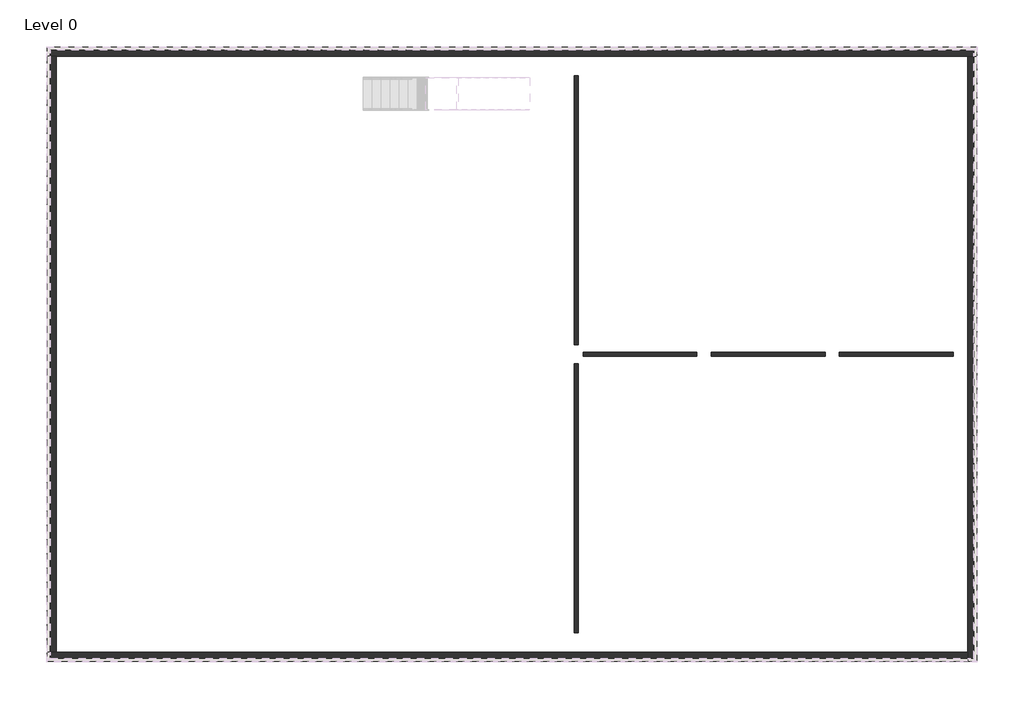
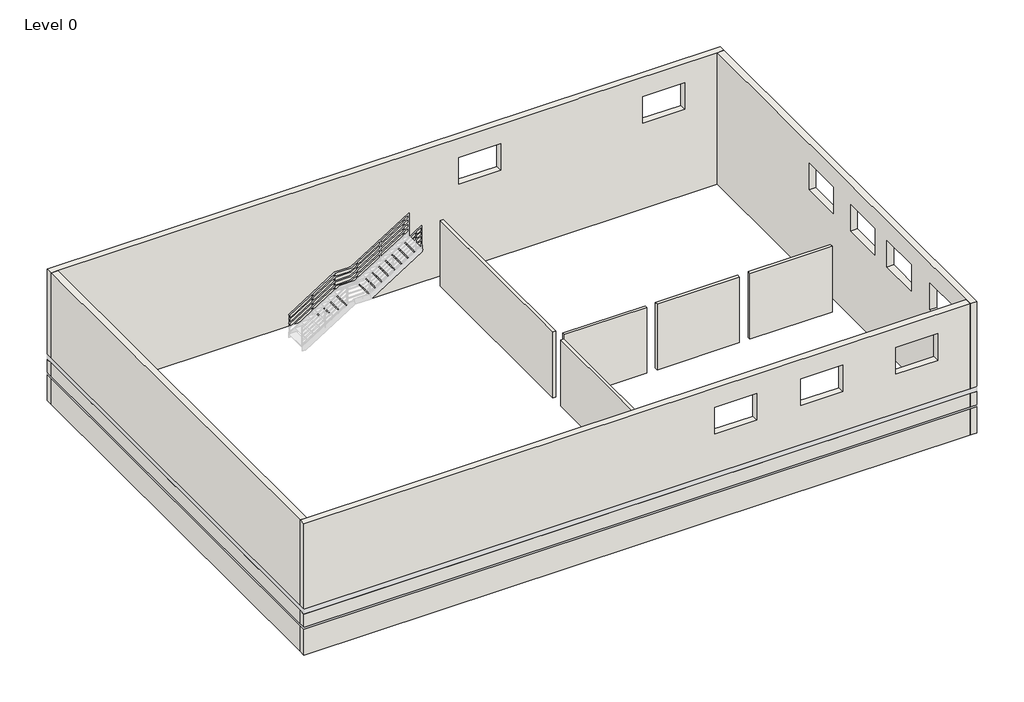
# One storey, part 1 of 3: 9 walls.
"""IFC4 building model written with IfcOpenShell, lengths in millimetres."""

from ifc_helpers import new_model, si_unit, frame, origin, origin_with_axes, place, context, project, spatial, polyline, outline, extrude, faceted_brep, element, save

model = new_model("IFC4")

# Units and contexts
model_context = context("Model", 3, world=origin())
ifc_project = project(units=[si_unit("LENGTHUNIT", "METRE", prefix="MILLI")], contexts=[model_context])

# Site, building, storey
site = spatial("IfcSite", under=ifc_project)
building = spatial("IfcBuilding", under=site)
storey = spatial("IfcBuildingStorey", under=building, Name="Level 0", Elevation=0.0)

# Walls
placement = place(None, origin())
element("IfcWall", 1, ObjectType="Wall-Ext_102Bwk-75Ins-100Blk-12P_Banding", at=placement, inside=storey, context=model_context, shape_type="Brep", body=[
    faceted_brep([(-15731.2051668, 9883.1317199, 0.0), (-15441.2051668, 9883.1317199, 0.0), (13008.7948332, 9883.1317199, 0.0), (13298.7948332, 9883.1317199, 0.0), (13298.7948332, 9883.1317199, 1200.0), (13216.2948332, 9883.1317199, 1200.0), (13216.2948332, 9883.1317199, 1275.0), (13298.7948332, 9883.1317199, 1275.0), (13298.7948332, 9883.1317199, 1885.0), (13196.7948332, 9883.1317199, 1885.0), (13196.7948332, 9883.1317199, 2110.0), (13298.7948332, 9883.1317199, 2110.0), (13298.7948332, 9883.1317199, 6000.0), (13008.7948332, 9883.1317199, 6000.0), (7058.7948332, 9883.1317199, 6000.0), (6958.7948332, 9883.1317199, 6000.0), (-15441.2051668, 9883.1317199, 6000.0), (-15731.2051668, 9883.1317199, 6000.0), (-15731.2051668, 9883.1317199, 2110.0), (-15629.2051668, 9883.1317199, 2110.0), (-15629.2051668, 9883.1317199, 1885.0), (-15731.2051668, 9883.1317199, 1885.0), (-15731.2051668, 9883.1317199, 1275.0), (-15648.7051668, 9883.1317199, 1275.0), (-15648.7051668, 9883.1317199, 1200.0), (-15731.2051668, 9883.1317199, 1200.0), (1848.7948332, 9883.1317199, 3900.0), (1848.7948332, 9883.1317199, 5110.0), (3658.7948332, 9883.1317199, 5110.0), (3658.7948332, 9883.1317199, 3900.0), (9798.7948332, 9883.1317199, 3900.0), (9798.7948332, 9883.1317199, 5110.0), (11608.7948332, 9883.1317199, 5110.0), (11608.7948332, 9883.1317199, 3900.0), (13298.7948332, 10173.1317199, 0.0), (-15731.2051668, 10173.1317199, 0.0), (-15731.2051668, 10173.1317199, 1200.0), (13298.7948332, 10173.1317199, 1200.0), (-15731.2051668, 10173.1317199, 6000.0), (13298.7948332, 10173.1317199, 6000.0), (13298.7948332, 10173.1317199, 2110.0), (-15731.2051668, 10173.1317199, 2110.0), (1848.7948332, 10173.1317199, 5110.0), (1848.7948332, 10173.1317199, 3900.0), (3658.7948332, 10173.1317199, 3900.0), (3658.7948332, 10173.1317199, 5110.0), (9798.7948332, 10173.1317199, 5110.0), (9798.7948332, 10173.1317199, 3900.0), (11608.7948332, 10173.1317199, 3900.0), (11608.7948332, 10173.1317199, 5110.0), (13298.7948332, 10173.1317199, 1275.0), (-15731.2051668, 10173.1317199, 1275.0), (-15731.2051668, 10173.1317199, 1885.0), (13298.7948332, 10173.1317199, 1885.0), (-15648.7051668, 10090.6317199, 1200.0), (-15648.7051668, 10090.6317199, 1275.0), (13216.2948332, 10090.6317199, 1275.0), (13216.2948332, 10090.6317199, 1200.0), (-15629.2051668, 10071.1317199, 1885.0), (-15629.2051668, 10071.1317199, 2110.0), (13196.7948332, 10071.1317199, 2110.0), (13196.7948332, 10071.1317199, 1885.0)], [[[0, 1, 2, 3, 4, 5, 6, 7, 8, 9, 10, 11, 12, 13, 14, 15, 16, 17, 18, 19, 20, 21, 22, 23, 24, 25], [26, 27, 28, 29], [30, 31, 32, 33]], [[34, 35, 36, 37]], [[38, 39, 40, 41], [42, 43, 44, 45], [46, 47, 48, 49]], [[50, 51, 52, 53]], [[3, 2, 1, 0, 35, 34]], [[17, 16, 15, 14, 13, 12, 39, 38]], [[54, 55, 56, 57]], [[58, 59, 60, 61]], [[3, 34, 37, 4]], [[39, 12, 11, 40]], [[7, 50, 53, 8]], [[57, 56, 6, 5]], [[61, 60, 10, 9]], [[17, 38, 41, 18]], [[35, 0, 25, 36]], [[51, 22, 21, 52]], [[55, 54, 24, 23]], [[56, 55, 23, 22, 51, 50, 7, 6]], [[54, 57, 5, 4, 37, 36, 25, 24]], [[59, 58, 20, 19]], [[60, 59, 19, 18, 41, 40, 11, 10]], [[58, 61, 9, 8, 53, 52, 21, 20]], [[43, 42, 27, 26]], [[44, 43, 26, 29]], [[45, 44, 29, 28]], [[42, 45, 28, 27]], [[47, 46, 31, 30]], [[48, 47, 30, 33]], [[49, 48, 33, 32]], [[46, 49, 32, 31]]]),
])
element("IfcWall", 2, ObjectType="Wall-Ext_102Bwk-75Ins-100Blk-12P_Banding", at=placement, inside=storey, context=model_context, shape_type="Brep", body=[
    faceted_brep([(13008.7948332, 9883.1317199, 0.0), (13008.7948332, -8716.8682801, 0.0), (13008.7948332, -9006.8682801, 0.0), (13008.7948332, -9006.8682801, 1200.0), (13008.7948332, -8924.3682801, 1200.0), (13008.7948332, -8924.3682801, 1275.0), (13008.7948332, -9006.8682801, 1275.0), (13008.7948332, -9006.8682801, 1885.0), (13008.7948332, -8904.8682801, 1885.0), (13008.7948332, -8904.8682801, 2110.0), (13008.7948332, -9006.8682801, 2110.0), (13008.7948332, -9006.8682801, 6000.0), (13008.7948332, -8716.8682801, 6000.0), (13008.7948332, 5333.1317199, 6000.0), (13008.7948332, 5433.1317199, 6000.0), (13008.7948332, 9883.1317199, 6000.0), (13008.7948332, -6006.8682801, 3900.0), (13008.7948332, -6006.8682801, 5110.0), (13008.7948332, -7816.8682801, 5110.0), (13008.7948332, -7816.8682801, 3900.0), (13008.7948332, -2796.8682801, 3900.0), (13008.7948332, -2796.8682801, 5110.0), (13008.7948332, -4606.8682801, 5110.0), (13008.7948332, -4606.8682801, 3900.0), (13008.7948332, -86.8682801, 3900.0), (13008.7948332, -86.8682801, 5110.0), (13008.7948332, -1896.8682801, 5110.0), (13008.7948332, -1896.8682801, 3900.0), (13008.7948332, 3023.1317199, 3900.0), (13008.7948332, 3023.1317199, 5110.0), (13008.7948332, 1213.1317199, 5110.0), (13008.7948332, 1213.1317199, 3900.0), (13298.7948332, -9006.8682801, 0.0), (13298.7948332, 9883.1317199, 0.0), (13298.7948332, 9883.1317199, 1200.0), (13298.7948332, -9006.8682801, 1200.0), (13298.7948332, 9883.1317199, 6000.0), (13298.7948332, -9006.8682801, 6000.0), (13298.7948332, -9006.8682801, 2110.0), (13298.7948332, 9883.1317199, 2110.0), (13298.7948332, -6006.8682801, 5110.0), (13298.7948332, -6006.8682801, 3900.0), (13298.7948332, -7816.8682801, 3900.0), (13298.7948332, -7816.8682801, 5110.0), (13298.7948332, -2796.8682801, 5110.0), (13298.7948332, -2796.8682801, 3900.0), (13298.7948332, -4606.8682801, 3900.0), (13298.7948332, -4606.8682801, 5110.0), (13298.7948332, -86.8682801, 5110.0), (13298.7948332, -86.8682801, 3900.0), (13298.7948332, -1896.8682801, 3900.0), (13298.7948332, -1896.8682801, 5110.0), (13298.7948332, 3023.1317199, 5110.0), (13298.7948332, 3023.1317199, 3900.0), (13298.7948332, 1213.1317199, 3900.0), (13298.7948332, 1213.1317199, 5110.0), (13298.7948332, -9006.8682801, 1275.0), (13298.7948332, 9883.1317199, 1275.0), (13298.7948332, 9883.1317199, 1885.0), (13298.7948332, -9006.8682801, 1885.0), (13216.2948332, -8924.3682801, 1200.0), (13216.2948332, 9883.1317199, 1200.0), (13216.2948332, 9883.1317199, 1275.0), (13216.2948332, -8924.3682801, 1275.0), (13196.7948332, -8904.8682801, 2110.0), (13196.7948332, -8904.8682801, 1885.0), (13196.7948332, 9883.1317199, 1885.0), (13196.7948332, 9883.1317199, 2110.0)], [[[0, 1, 2, 3, 4, 5, 6, 7, 8, 9, 10, 11, 12, 13, 14, 15], [16, 17, 18, 19], [20, 21, 22, 23], [24, 25, 26, 27], [28, 29, 30, 31]], [[32, 33, 34, 35]], [[36, 37, 38, 39], [40, 41, 42, 43], [44, 45, 46, 47], [48, 49, 50, 51], [52, 53, 54, 55]], [[56, 57, 58, 59]], [[2, 1, 0, 33, 32]], [[15, 14, 13, 12, 11, 37, 36]], [[60, 61, 62, 63]], [[64, 65, 66, 67]], [[0, 15, 36, 39, 67, 66, 58, 57, 62, 61, 34, 33]], [[63, 62, 57, 56, 6, 5]], [[61, 60, 4, 3, 35, 34]], [[9, 64, 67, 39, 38, 10]], [[66, 65, 8, 7, 59, 58]], [[2, 32, 35, 3]], [[37, 11, 10, 38]], [[6, 56, 59, 7]], [[60, 63, 5, 4]], [[65, 64, 9, 8]], [[41, 40, 17, 16]], [[42, 41, 16, 19]], [[43, 42, 19, 18]], [[40, 43, 18, 17]], [[45, 44, 21, 20]], [[46, 45, 20, 23]], [[47, 46, 23, 22]], [[44, 47, 22, 21]], [[49, 48, 25, 24]], [[50, 49, 24, 27]], [[51, 50, 27, 26]], [[48, 51, 26, 25]], [[53, 52, 29, 28]], [[54, 53, 28, 31]], [[55, 54, 31, 30]], [[52, 55, 30, 29]]]),
])
element("IfcWall", 3, ObjectType="Wall-Ext_102Bwk-75Ins-100Blk-12P_Banding", at=placement, inside=storey, context=model_context, shape_type="Brep", body=[
    faceted_brep([(13008.7948332, -8716.8682801, 0.0), (-15441.2051668, -8716.8682801, 0.0), (-15731.2051668, -8716.8682801, 0.0), (-15731.2051668, -8716.8682801, 1200.0), (-15648.7051668, -8716.8682801, 1200.0), (-15648.7051668, -8716.8682801, 1275.0), (-15731.2051668, -8716.8682801, 1275.0), (-15731.2051668, -8716.8682801, 1885.0), (-15629.2051668, -8716.8682801, 1885.0), (-15629.2051668, -8716.8682801, 2110.0), (-15731.2051668, -8716.8682801, 2110.0), (-15731.2051668, -8716.8682801, 6000.0), (-15441.2051668, -8716.8682801, 6000.0), (13008.7948332, -8716.8682801, 6000.0), (3808.7948332, -8716.8682801, 3900.0), (3808.7948332, -8716.8682801, 5110.0), (1998.7948332, -8716.8682801, 5110.0), (1998.7948332, -8716.8682801, 3900.0), (7518.7948332, -8716.8682801, 3900.0), (7518.7948332, -8716.8682801, 5110.0), (5708.7948332, -8716.8682801, 5110.0), (5708.7948332, -8716.8682801, 3900.0), (11608.7948332, -8716.8682801, 3900.0), (11608.7948332, -8716.8682801, 5110.0), (9798.7948332, -8716.8682801, 5110.0), (9798.7948332, -8716.8682801, 3900.0), (-15731.2051668, -9006.8682801, 0.0), (13008.7948332, -9006.8682801, 0.0), (13008.7948332, -9006.8682801, 1200.0), (-15731.2051668, -9006.8682801, 1200.0), (13008.7948332, -9006.8682801, 6000.0), (-15731.2051668, -9006.8682801, 6000.0), (-15731.2051668, -9006.8682801, 2110.0), (13008.7948332, -9006.8682801, 2110.0), (3808.7948332, -9006.8682801, 5110.0), (3808.7948332, -9006.8682801, 3900.0), (1998.7948332, -9006.8682801, 3900.0), (1998.7948332, -9006.8682801, 5110.0), (7518.7948332, -9006.8682801, 5110.0), (7518.7948332, -9006.8682801, 3900.0), (5708.7948332, -9006.8682801, 3900.0), (5708.7948332, -9006.8682801, 5110.0), (11608.7948332, -9006.8682801, 5110.0), (11608.7948332, -9006.8682801, 3900.0), (9798.7948332, -9006.8682801, 3900.0), (9798.7948332, -9006.8682801, 5110.0), (-15731.2051668, -9006.8682801, 1275.0), (13008.7948332, -9006.8682801, 1275.0), (13008.7948332, -9006.8682801, 1885.0), (-15731.2051668, -9006.8682801, 1885.0), (-15648.7051668, -8924.3682801, 1200.0), (13008.7948332, -8924.3682801, 1200.0), (13008.7948332, -8924.3682801, 1275.0), (-15648.7051668, -8924.3682801, 1275.0), (-15629.2051668, -8904.8682801, 2110.0), (-15629.2051668, -8904.8682801, 1885.0), (13008.7948332, -8904.8682801, 1885.0), (13008.7948332, -8904.8682801, 2110.0)], [[[0, 1, 2, 3, 4, 5, 6, 7, 8, 9, 10, 11, 12, 13], [14, 15, 16, 17], [18, 19, 20, 21], [22, 23, 24, 25]], [[26, 27, 28, 29]], [[30, 31, 32, 33], [34, 35, 36, 37], [38, 39, 40, 41], [42, 43, 44, 45]], [[46, 47, 48, 49]], [[2, 1, 0, 27, 26]], [[13, 12, 11, 31, 30]], [[50, 51, 52, 53]], [[54, 55, 56, 57]], [[0, 13, 30, 33, 57, 56, 48, 47, 52, 51, 28, 27]], [[53, 52, 47, 46, 6, 5]], [[51, 50, 4, 3, 29, 28]], [[9, 54, 57, 33, 32, 10]], [[56, 55, 8, 7, 49, 48]], [[2, 26, 29, 3]], [[31, 11, 10, 32]], [[6, 46, 49, 7]], [[50, 53, 5, 4]], [[55, 54, 9, 8]], [[35, 34, 15, 14]], [[36, 35, 14, 17]], [[37, 36, 17, 16]], [[34, 37, 16, 15]], [[39, 38, 19, 18]], [[40, 39, 18, 21]], [[41, 40, 21, 20]], [[38, 41, 20, 19]], [[43, 42, 23, 22]], [[44, 43, 22, 25]], [[45, 44, 25, 24]], [[42, 45, 24, 23]]]),
])
element("IfcWall", 4, ObjectType="Wall-Ext_102Bwk-75Ins-100Blk-12P_Banding", at=placement, inside=storey, context=model_context, shape_type="SweptSolid", body=[
    extrude(outline(polyline([(0.0, -15441.2051668), (6000.0, -15441.2051668), (6000.0, -15731.2051668), (2110.0, -15731.2051668), (2110.0, -15629.2051668), (1885.0, -15629.2051668), (1885.0, -15731.2051668), (1275.0, -15731.2051668), (1275.0, -15648.7051668), (1200.0, -15648.7051668), (1200.0, -15731.2051668), (0.0, -15731.2051668), (0.0, -15441.2051668)])), frame((0.0, -8716.8682801, 0.0), z_axis=(0.0, 1.0, 0.0), x_axis=(0.0, 0.0, 1.0)), (0.0, 0.0, 1.0), 18600.0),
])
element("IfcWall", 5, ObjectType="Wall-Int_12P-100Blk-12P", at=placement, inside=storey, context=model_context, shape_type="SweptSolid", body=[
    extrude(outline(polyline([(846.2948332, 283.1317199), (846.2948332, -8116.8682801), (721.2948332, -8116.8682801), (721.2948332, 283.1317199), (846.2948332, 283.1317199)])), origin_with_axes(), (0.0, 0.0, 1.0), 3000.0),
])
element("IfcWall", 6, ObjectType="Wall-Int_12P-100Blk-12P", at=placement, inside=storey, context=model_context, shape_type="SweptSolid", body=[
    extrude(outline(polyline([(846.2948332, 9283.1317199), (846.2948332, 883.1317199), (721.2948332, 883.1317199), (721.2948332, 9283.1317199), (846.2948332, 9283.1317199)])), origin_with_axes(), (0.0, 0.0, 1.0), 3000.0),
])
element("IfcWall", 7, ObjectType="Wall-Int_12P-100Blk-12P", at=placement, inside=storey, context=model_context, shape_type="SweptSolid", body=[
    extrude(outline(polyline([(4558.7948332, 520.6317199), (1008.7948332, 520.6317199), (1008.7948332, 645.6317199), (4558.7948332, 645.6317199), (4558.7948332, 520.6317199)])), origin_with_axes(), (0.0, 0.0, 1.0), 3000.0),
])
element("IfcWall", 8, ObjectType="Wall-Int_12P-100Blk-12P", at=placement, inside=storey, context=model_context, shape_type="SweptSolid", body=[
    extrude(outline(polyline([(5008.7948332, 645.6317199), (8558.7948332, 645.6317199), (8558.7948332, 520.6317199), (5008.7948332, 520.6317199), (5008.7948332, 645.6317199)])), origin_with_axes(), (0.0, 0.0, 1.0), 3000.0),
])
element("IfcWall", 9, ObjectType="Wall-Int_12P-100Blk-12P", at=placement, inside=storey, context=model_context, shape_type="SweptSolid", body=[
    extrude(outline(polyline([(9008.7948332, 645.6317199), (12558.7948332, 645.6317199), (12558.7948332, 520.6317199), (9008.7948332, 520.6317199), (9008.7948332, 645.6317199)])), origin_with_axes(), (0.0, 0.0, 1.0), 3000.0),
])

save(model, "model.ifc")

# Revit data of these elements
# Project information
#   Project Issue Date = "Issue Date"
#   Project Status = "Project Status"
#   Client Name = "Owner"
#   Project Address = "Enter address here"
#   Project Name = "Project Name"
#   Project Number = "Project Number"
# Type "Wall-Ext_102Bwk-75Ins-100Blk-12P_Banding"
#   Keynote = "F10"
#   Layers, outside or top first: 102.5 mm "Brick, Engineering, Grey" (function 4); 102.5 mm "Brick, Horizontal Pattern" (function 4); 75 mm "Fiberglass Batt" (function 3); 100 mm "Concrete Masonry Units" (function 1); 12.5 mm "Plaster" (function 5)
# Type "Wall-Int_12P-100Blk-12P"
#   Layers, outside or top first: 12.5 mm "Plaster" (function 5); 100 mm "Concrete Masonry Units" (function 1); 12.5 mm "Plaster" (function 5)
# Elements 1, 2, 3 (IfcWall, "Wall-Ext_102Bwk-75Ins-100Blk-12P_Banding")
#   Top Offset = 0 mm
#   Base Offset = 0 mm
#   wall height = 6000 mm
#   Phase Created = New Construction
#   Base Constraint = Level 0
#   Top Constraint = Level 2
#   Materials on its faces: "Default Wall", "Brick, Horizontal Pattern", "Brick, Engineering, Grey", "Plaster"
# Element 4 (IfcWall, "Wall-Ext_102Bwk-75Ins-100Blk-12P_Banding")
#   Top Offset = 0 mm
#   Base Offset = 0 mm
#   wall height = 6000 mm
#   Phase Created = New Construction
#   Base Constraint = Level 0
#   Top Constraint = Level 2
#   Materials on its faces: "Brick, Horizontal Pattern", "Default Wall", "Plaster", "Brick, Engineering, Grey"
# Elements 5, 6, 7, 8, 9 (IfcWall, "Wall-Int_12P-100Blk-12P")
#   Top Offset = 0 mm
#   Base Offset = 0 mm
#   wall height = 3000 mm
#   Phase Created = New Construction
#   Base Constraint = Level 0
#   Top Constraint = Level 1
#   Materials on its faces: "Default Wall", "Plaster"
# Materials
#   "Brick, Engineering, Grey": class "Masonry", colour RGB 205 205 205, transparency 0, Description = "High fired, dense brick", Cost = 0
#   "Brick, Horizontal Pattern": class "Masonry", colour RGB 216 173 168, transparency 0, Description = "physical material", Cost = 0
#   "Fiberglass Batt": class "Generic", colour RGB 127 127 127, transparency 0, Description = "Fiberglass batt insulation", Cost = 0
#   "Concrete Masonry Units": class "Masonry", colour RGB 181 181 181, transparency 0, Description = "Concrete masonry units", Cost = 0
#   "Plaster": class "Generic", colour RGB 249 249 249, transparency 0, Description = "Plaster", Cost = 0
#   "Default Wall": class "Miscellaneous", colour RGB 128 128 128, transparency 0, Comments = "Rendering appearance not upgraded ", Cost = 0
